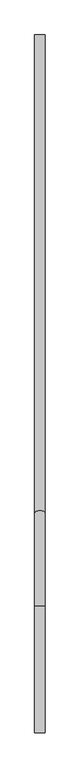
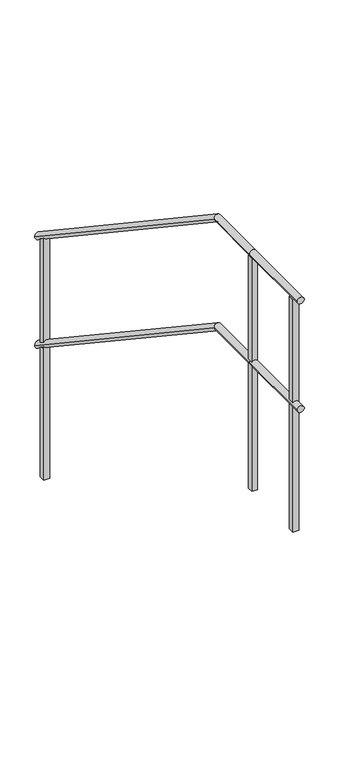
"""IFC4 building model written with IfcOpenShell, lengths in millimetres: railing geometry."""

from ifc_helpers import new_model, si_unit, frame, origin, place, context, project, spatial, polyline, circle_curve, ellipse_curve, outline, extrude, source, transform, mapped, element, save
from ifc_brep_helpers import plane_surface, cylinder_surface, advanced_brep


def railing_b278a75e(model_context):
    return source(origin(), model_context, "Body", "SolidModel", [
        advanced_brep(
        [(13536.7845799, 439.5208589, 9484.9618634), (13566.7845799, 439.5208589, 9484.9618634), (13536.7845799, 799.5208589, 9484.9618634), (13566.7845799, 799.5208589, 9484.9618634)],
        [
            (0, 1, circle_curve(frame((13551.7845799, 439.5208589, 9484.9618634), z_axis=(0.0, -1.0, 0.0), x_axis=(1.0, 0.0, 0.0)), 15.0)),
            (1, 0, circle_curve(frame((13551.7845799, 439.5208589, 9484.9618634), z_axis=(0.0, -1.0, 0.0), x_axis=(1.0, 0.0, 0.0)), 15.0)),
            (2, 3, circle_curve(frame((13551.7845799, 799.5208589, 9484.9618634), z_axis=(0.0, 1.0, 0.0), x_axis=(1.0, 0.0, 0.0)), 15.0)),
            (3, 2, circle_curve(frame((13551.7845799, 799.5208589, 9484.9618634), z_axis=(0.0, 1.0, 0.0), x_axis=(1.0, 0.0, 0.0)), 15.0)),
            (0, 2),
            (3, 1),
        ],
        [
            plane_surface(frame((13551.7845799, 439.5208589, 9499.9618634), z_axis=(0.0, -1.0, 0.0), x_axis=(0.0, 0.0, 1.0))),
            plane_surface(frame((13551.7845799, 799.5208589, 9499.9618634), z_axis=(0.0, 1.0, 0.0), x_axis=(0.0, 0.0, 1.0))),
            cylinder_surface(frame((13551.7845799, 439.5208589, 9484.9618634), z_axis=(0.0, -1.0, 0.0), x_axis=(1.0, 0.0, 0.0)), 15.0),
        ],
        [
            (0, [[1, 2]]),
            (1, [[3, 4]]),
            (2, [[-1, 5, -4, 6]]),
            (2, [[-2, -6, -3, -5]]),
        ],
    ),
        advanced_brep(
        [(13536.7845799, 799.5208589, 9484.9618634), (13566.7845799, 799.5208589, 9484.9618634), (13536.7845799, 1064.9792243, 9484.9618634), (13566.7845799, 1064.9792243, 9484.9618634), (13536.7845799, 2419.5208589, 8581.934107), (13566.7845799, 2419.5208589, 8581.934107)],
        [
            (0, 1, circle_curve(frame((13551.7845799, 799.5208589, 9484.9618634), z_axis=(0.0, -1.0, 0.0), x_axis=(1.0, 0.0, 0.0)), 15.0)),
            (1, 0, circle_curve(frame((13551.7845799, 799.5208589, 9484.9618634), z_axis=(0.0, -1.0, 0.0), x_axis=(1.0, 0.0, 0.0)), 15.0)),
            (0, 2),
            (2, 3, ellipse_curve(frame((13551.7845799, 1064.9792243, 9484.9618634), z_axis=(0.0, -0.9570920264890528, 0.28978414868843017), x_axis=(0.0, -0.2897841486884305, -0.9570920264890528)), 15.6724741, 15.0)),
            (3, 1),
            (3, 2, ellipse_curve(frame((13551.7845799, 1064.9792243, 9484.9618634), z_axis=(0.0, -0.9570920264890528, 0.28978414868843017), x_axis=(0.0, -0.2897841486884305, -0.9570920264890528)), 15.6724741, 15.0)),
            (4, 5, ellipse_curve(frame((13551.7845799, 2419.5208589, 8581.934107), z_axis=(0.0, 1.0, 0.0), x_axis=(0.0, 0.0, 1.0)), 18.0277564, 15.0)),
            (5, 4, ellipse_curve(frame((13551.7845799, 2419.5208589, 8581.934107), z_axis=(0.0, 1.0, 0.0), x_axis=(0.0, 0.0, 1.0)), 18.0277564, 15.0)),
            (2, 4),
            (5, 3),
        ],
        [
            plane_surface(frame((13551.7845799, 799.5208589, 9499.9618634), z_axis=(0.0, -1.0, 0.0), x_axis=(0.0, 0.0, 1.0))),
            cylinder_surface(frame((13551.7845799, 799.5208589, 9484.9618634), z_axis=(0.0, -1.0, 0.0), x_axis=(1.0, 0.0, 0.0)), 15.0),
            plane_surface(frame((13551.7845799, 2419.5208589, 8599.9618634), z_axis=(0.0, 1.0, 0.0), x_axis=(0.0, 0.0, 1.0))),
            cylinder_surface(frame((13551.7845799, 1061.2003559, 9487.481109), z_axis=(0.0, -0.8320502943378436, 0.5547001962252293), x_axis=(1.0, 0.0, 0.0)), 15.0),
        ],
        [
            (0, [[1, 2]]),
            (1, [[-1, 3, 4, 5]]),
            (1, [[-2, -5, 6, -3]]),
            (2, [[7, 8]]),
            (3, [[-4, 9, -8, 10]]),
            (3, [[-6, -10, -7, -9]]),
        ],
    ),
        advanced_brep(
        [(13536.7845799, 439.5208589, 9984.9618634), (13566.7845799, 439.5208589, 9984.9618634), (13536.7845799, 799.5208589, 9984.9618634), (13566.7845799, 799.5208589, 9984.9618634)],
        [
            (0, 1, circle_curve(frame((13551.7845799, 439.5208589, 9984.9618634), z_axis=(0.0, -1.0, 0.0), x_axis=(1.0, 0.0, 0.0)), 15.0)),
            (1, 0, circle_curve(frame((13551.7845799, 439.5208589, 9984.9618634), z_axis=(0.0, -1.0, 0.0), x_axis=(1.0, 0.0, 0.0)), 15.0)),
            (2, 3, circle_curve(frame((13551.7845799, 799.5208589, 9984.9618634), z_axis=(0.0, 1.0, 0.0), x_axis=(1.0, 0.0, 0.0)), 15.0)),
            (3, 2, circle_curve(frame((13551.7845799, 799.5208589, 9984.9618634), z_axis=(0.0, 1.0, 0.0), x_axis=(1.0, 0.0, 0.0)), 15.0)),
            (0, 2),
            (3, 1),
        ],
        [
            plane_surface(frame((13551.7845799, 439.5208589, 9999.9618634), z_axis=(0.0, -1.0, 0.0), x_axis=(0.0, 0.0, 1.0))),
            plane_surface(frame((13551.7845799, 799.5208589, 9999.9618634), z_axis=(0.0, 1.0, 0.0), x_axis=(0.0, 0.0, 1.0))),
            cylinder_surface(frame((13551.7845799, 439.5208589, 9984.9618634), z_axis=(0.0, -1.0, 0.0), x_axis=(1.0, 0.0, 0.0)), 15.0),
        ],
        [
            (0, [[1, 2]]),
            (1, [[3, 4]]),
            (2, [[-1, 5, -4, 6]]),
            (2, [[-2, -6, -3, -5]]),
        ],
    ),
        advanced_brep(
        [(13536.7845799, 799.5208589, 9984.9618634), (13566.7845799, 799.5208589, 9984.9618634), (13536.7845799, 1064.9792243, 9984.9618634), (13566.7845799, 1064.9792243, 9984.9618634), (13536.7845799, 2419.5208589, 9081.934107), (13566.7845799, 2419.5208589, 9081.934107)],
        [
            (0, 1, circle_curve(frame((13551.7845799, 799.5208589, 9984.9618634), z_axis=(0.0, -1.0, 0.0), x_axis=(1.0, 0.0, 0.0)), 15.0)),
            (1, 0, circle_curve(frame((13551.7845799, 799.5208589, 9984.9618634), z_axis=(0.0, -1.0, 0.0), x_axis=(1.0, 0.0, 0.0)), 15.0)),
            (0, 2),
            (2, 3, ellipse_curve(frame((13551.7845799, 1064.9792243, 9984.9618634), z_axis=(0.0, -0.9570920264890528, 0.28978414868843017), x_axis=(0.0, -0.2897841486884305, -0.9570920264890528)), 15.6724741, 15.0)),
            (3, 1),
            (3, 2, ellipse_curve(frame((13551.7845799, 1064.9792243, 9984.9618634), z_axis=(0.0, -0.9570920264890528, 0.28978414868843017), x_axis=(0.0, -0.2897841486884305, -0.9570920264890528)), 15.6724741, 15.0)),
            (4, 5, ellipse_curve(frame((13551.7845799, 2419.5208589, 9081.934107), z_axis=(0.0, 1.0, 0.0), x_axis=(0.0, 0.0, 1.0)), 18.0277564, 15.0)),
            (5, 4, ellipse_curve(frame((13551.7845799, 2419.5208589, 9081.934107), z_axis=(0.0, 1.0, 0.0), x_axis=(0.0, 0.0, 1.0)), 18.0277564, 15.0)),
            (2, 4),
            (5, 3),
        ],
        [
            plane_surface(frame((13551.7845799, 799.5208589, 9999.9618634), z_axis=(0.0, -1.0, 0.0), x_axis=(0.0, 0.0, 1.0))),
            cylinder_surface(frame((13551.7845799, 799.5208589, 9984.9618634), z_axis=(0.0, -1.0, 0.0), x_axis=(1.0, 0.0, 0.0)), 15.0),
            plane_surface(frame((13551.7845799, 2419.5208589, 9099.9618634), z_axis=(0.0, 1.0, 0.0), x_axis=(0.0, 0.0, 1.0))),
            cylinder_surface(frame((13551.7845799, 1061.2003559, 9987.481109), z_axis=(0.0, -0.8320502943378436, 0.5547001962252293), x_axis=(1.0, 0.0, 0.0)), 15.0),
        ],
        [
            (0, [[1, 2]]),
            (1, [[-1, 3, 4, 5]]),
            (1, [[-2, -5, 6, -3]]),
            (2, [[7, 8]]),
            (3, [[-4, 9, -8, 10]]),
            (3, [[-6, -10, -7, -9]]),
        ],
    ),
        extrude(outline(polyline([(13564.2845799, 787.0208589), (13539.2845799, 787.0208589), (13539.2845799, 812.0208589), (13564.2845799, 812.0208589), (13564.2845799, 787.0208589)])), frame((0.0, 0.0, 8899.9618634), z_axis=(0.0, 0.0, 1.0), x_axis=(1.0, 0.0, 0.0)), (0.0, 0.0, 1.0), 1070.0),
        extrude(outline(polyline([(2357.0208589, 7999.9618634), (2357.0208589, 9111.62853), (2382.0208589, 9094.9618634), (2382.0208589, 7999.9618634), (2357.0208589, 7999.9618634)])), frame((13539.2845799, 0.0, 0.0), z_axis=(1.0, 0.0, 0.0), x_axis=(0.0, 1.0, 0.0)), (0.0, 0.0, 1.0), 25.0),
        extrude(outline(polyline([(13564.2845799, 477.0208589), (13539.2845799, 477.0208589), (13539.2845799, 502.0208589), (13564.2845799, 502.0208589), (13564.2845799, 477.0208589)])), frame((0.0, 0.0, 8899.9618634), z_axis=(0.0, 0.0, 1.0), x_axis=(1.0, 0.0, 0.0)), (0.0, 0.0, 1.0), 1070.0),
    ])


if __name__ == "__main__":
    model = new_model("IFC4")
    model_context = context("Model", 3, world=origin())
    ifc_project = project(units=[si_unit("LENGTHUNIT", "METRE", prefix="MILLI")], contexts=[model_context])
    site = spatial("IfcSite", under=ifc_project)
    building = spatial("IfcBuilding", under=site)
    placement = place(None, origin())
    railing_shape = railing_b278a75e(model_context)
    element("IfcRailing", 1, at=placement, inside=building, context=model_context, shape_type="MappedRepresentation", body=[
        mapped(railing_shape, transform((0.0, 0.0, 0.0), x_axis=(1.0, 0.0, 0.0), y_axis=(0.0, 1.0, 0.0), z_axis=(0.0, 0.0, 1.0))),
    ])
    save(model, "model.ifc")
